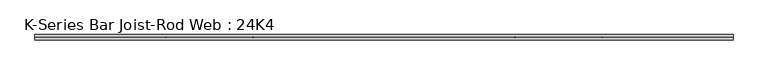
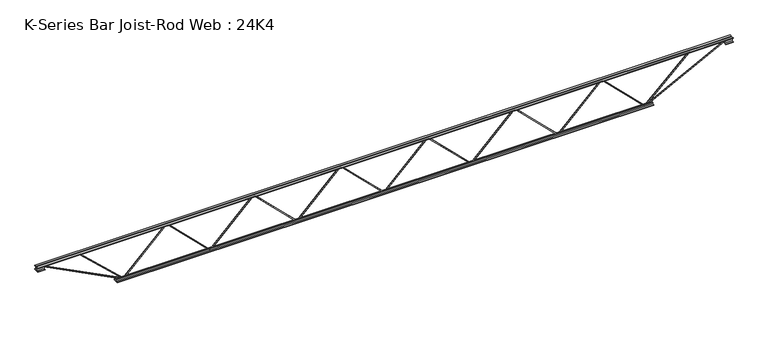
"""IFC4 building model written with IfcOpenShell, lengths in millimetres: beam geometry, K-Series Bar Joist-Rod Web : 24K4."""

from ifc_helpers import new_model, si_unit, frame, origin, place, context, project, spatial, polyline, outline, extrude, source, transform, mapped, element, save


def k_series_bar_joist_rod_web_24k4_b54f82ce(model_context):
    return source(origin(), model_context, "Body", "SweptSolid", [
        extrude(outline(polyline([(-293.6875, 1223.645), (-303.2125, 1223.645), (-303.2125, 1228.7733784), (293.6875, 1834.0077534), (293.6875, 1836.4509966), (-303.2125, 2441.6853716), (-303.2125, 2446.81375), (-293.6875, 2446.81375), (-293.6875, 2445.5921284), (303.2125, 1840.3577534), (303.2125, 1830.1009966), (-293.6875, 1224.8666216), (-293.6875, 1223.645)])), frame((0.0, -4.7625, 0.0), z_axis=(0.0, 1.0, 0.0), x_axis=(0.0, 0.0, 1.0)), (0.0, 0.0, 1.0), 9.525),
        extrude(outline(polyline([(-293.6875, 0.15875), (-303.2125, 0.15875), (-303.2125, 5.2871284), (293.6875, 610.5215034), (293.6875, 612.9647466), (-303.2125, 1218.1991216), (-303.2125, 1223.3275), (-293.6875, 1223.3275), (-293.6875, 1222.1058784), (303.2125, 616.8715034), (303.2125, 606.6147466), (-293.6875, 1.3803716), (-293.6875, 0.15875)])), frame((0.0, -4.7625, 0.0), z_axis=(0.0, 1.0, 0.0), x_axis=(0.0, 0.0, 1.0)), (0.0, 0.0, 1.0), 9.525),
        extrude(outline(polyline([(-293.6875, -1223.3275), (-303.2125, -1223.3275), (-303.2125, -1218.1991216), (293.6875, -612.9647466), (293.6875, -610.5215034), (-303.2125, -5.2871284), (-303.2125, -0.15875), (-293.6875, -0.15875), (-293.6875, -1.3803716), (303.2125, -606.6147466), (303.2125, -616.8715034), (-293.6875, -1222.1058784), (-293.6875, -1223.3275)])), frame((0.0, -4.7625, 0.0), z_axis=(0.0, 1.0, 0.0), x_axis=(0.0, 0.0, 1.0)), (0.0, 0.0, 1.0), 9.525),
        extrude(outline(polyline([(-293.6875, -2446.81375), (-303.2125, -2446.81375), (-303.2125, -2441.6853716), (293.6875, -1836.4509966), (293.6875, -1834.0077534), (-303.2125, -1228.7733784), (-303.2125, -1223.645), (-293.6875, -1223.645), (-293.6875, -1224.8666216), (303.2125, -1830.1009966), (303.2125, -1840.3577534), (-293.6875, -2445.5921284), (-293.6875, -2446.81375)])), frame((0.0, -4.7625, 0.0), z_axis=(0.0, 1.0, 0.0), x_axis=(0.0, 0.0, 1.0)), (0.0, 0.0, 1.0), 9.525),
        extrude(outline(polyline([(-293.6875, 2447.13125), (-303.2125, 2447.13125), (-303.2125, 2452.2596284), (293.6875, 3057.4940034), (293.6875, 3059.9372466), (-303.2125, 3665.1716216), (-303.2125, 3670.3), (-293.6875, 3670.3), (-293.6875, 3669.0783784), (303.2125, 3063.8440034), (303.2125, 3053.5872466), (-293.6875, 2448.3528716), (-293.6875, 2447.13125)])), frame((0.0, -4.7625, 0.0), z_axis=(0.0, 1.0, 0.0), x_axis=(0.0, 0.0, 1.0)), (0.0, 0.0, 1.0), 9.525),
        extrude(outline(polyline([(-293.6875, -3670.3), (-303.2125, -3670.3), (-303.2125, -3665.1716216), (293.6875, -3059.9372466), (293.6875, -3057.4940034), (-303.2125, -2452.2596284), (-303.2125, -2447.13125), (-293.6875, -2447.13125), (-293.6875, -2448.3528716), (303.2125, -3053.5872466), (303.2125, -3063.8440034), (-293.6875, -3669.0783784), (-293.6875, -3670.3)])), frame((0.0, -4.7625, 0.0), z_axis=(0.0, 1.0, 0.0), x_axis=(0.0, 0.0, 1.0)), (0.0, 0.0, 1.0), 9.525),
        extrude(outline(polyline([(4.7625, 304.8), (36.5125, 304.8), (36.5125, 298.45), (11.1125, 298.45), (11.1125, 273.05), (4.7625, 273.05), (4.7625, 304.8)])), frame((-4889.5, 0.0, 0.0), z_axis=(1.0, 0.0, 0.0), x_axis=(0.0, 1.0, 0.0)), (0.0, 0.0, 1.0), 9779.0),
        extrude(outline(polyline([(-4.7625, 304.8), (-4.7625, 273.05), (-11.1125, 273.05), (-11.1125, 298.45), (-36.5125, 298.45), (-36.5125, 304.8), (-4.7625, 304.8)])), frame((-4889.5, 0.0, 0.0), z_axis=(1.0, 0.0, 0.0), x_axis=(0.0, 1.0, 0.0)), (0.0, 0.0, 1.0), 9779.0),
        extrude(outline(polyline([(-4.7625, 241.3), (-36.5125, 241.3), (-36.5125, 247.65), (-11.1125, 247.65), (-11.1125, 273.05), (-4.7625, 273.05), (-4.7625, 241.3)])), frame((-4889.5, 0.0, 0.0), z_axis=(1.0, 0.0, 0.0), x_axis=(0.0, 1.0, 0.0)), (0.0, 0.0, 1.0), 101.6),
        extrude(outline(polyline([(36.5125, 241.3), (4.7625, 241.3), (4.7625, 273.05), (11.1125, 273.05), (11.1125, 247.65), (36.5125, 247.65), (36.5125, 241.3)])), frame((-4889.5, 0.0, 0.0), z_axis=(1.0, 0.0, 0.0), x_axis=(0.0, 1.0, 0.0)), (0.0, 0.0, 1.0), 101.6),
        extrude(outline(polyline([(4.7625, 241.3), (4.7625, 273.05), (11.1125, 273.05), (11.1125, 247.65), (36.5125, 247.65), (36.5125, 241.3), (4.7625, 241.3)])), frame((4787.9, 0.0, 0.0), z_axis=(1.0, 0.0, 0.0), x_axis=(0.0, 1.0, 0.0)), (0.0, 0.0, 1.0), 101.6),
        extrude(outline(polyline([(-4.7625, 241.3), (-36.5125, 241.3), (-36.5125, 247.65), (-11.1125, 247.65), (-11.1125, 273.05), (-4.7625, 273.05), (-4.7625, 241.3)])), frame((4787.9, 0.0, 0.0), z_axis=(1.0, 0.0, 0.0), x_axis=(0.0, 1.0, 0.0)), (0.0, 0.0, 1.0), 101.6),
        extrude(outline(polyline([(4.7625, -304.8), (4.7625, -273.05), (11.1125, -273.05), (11.1125, -298.45), (36.5125, -298.45), (36.5125, -304.8), (4.7625, -304.8)])), frame((-3771.9, 0.0, 0.0), z_axis=(1.0, 0.0, 0.0), x_axis=(0.0, 1.0, 0.0)), (0.0, 0.0, 1.0), 7543.8),
        extrude(outline(polyline([(-4.7625, -304.8), (-36.5125, -304.8), (-36.5125, -298.45), (-11.1125, -298.45), (-11.1125, -273.05), (-4.7625, -273.05), (-4.7625, -304.8)])), frame((-3771.9, 0.0, 0.0), z_axis=(1.0, 0.0, 0.0), x_axis=(0.0, 1.0, 0.0)), (0.0, 0.0, 1.0), 7543.8),
        extrude(outline(polyline([(0.0, -9.525), (0.0, 0.0), (1255.2457966, 0.0), (1255.2457966, -9.525), (0.0, -9.525)])), frame((-4790.0683154, 4.7625, 268.8097388), z_axis=(0.4552893158665215, 0.0, 0.8903435510283628), x_axis=(0.8903435510283628, 0.0, -0.4552893158665215)), (0.0, 0.0, 1.0), 9.525),
        extrude(outline(polyline([(0.0, -9.525), (0.0, 0.0), (837.0470105, 0.0), (837.0470105, -9.525), (0.0, -9.525)])), frame((-4285.1360069, 4.7625, 269.5703023), z_axis=(0.6827573515565594, 0.0, 0.7306451935758373), x_axis=(0.7306451935758373, 0.0, -0.6827573515565594)), (0.0, 0.0, 1.0), 9.525),
        extrude(outline(polyline([(0.0, -9.525), (0.0, 0.0), (1255.2457966, 0.0), (1255.2457966, -9.525), (0.0, -9.525)])), frame((4790.0683154, -4.7625, 268.8097388), z_axis=(-0.455289315866513, 0.0, 0.8903435510283672), x_axis=(-0.8903435510283672, 0.0, -0.455289315866513)), (0.0, 0.0, 1.0), 9.525),
        extrude(outline(polyline([(0.0, -9.525), (0.0, 0.0), (837.0470105, 0.0), (837.0470105, -9.525), (0.0, -9.525)])), frame((4285.1360069, -4.7625, 269.5703023), z_axis=(-0.6827573515565561, 0.0, 0.7306451935758403), x_axis=(-0.7306451935758403, 0.0, -0.6827573515565561)), (0.0, 0.0, 1.0), 9.525),
    ])


if __name__ == "__main__":
    model = new_model("IFC4")
    model_context = context("Model", 3, world=origin())
    ifc_project = project(units=[si_unit("LENGTHUNIT", "METRE", prefix="MILLI")], contexts=[model_context])
    site = spatial("IfcSite", under=ifc_project)
    building = spatial("IfcBuilding", under=site)
    placement = place(None, origin())
    k_series_bar_joist_rod_web_24k4_shape = k_series_bar_joist_rod_web_24k4_b54f82ce(model_context)
    element("IfcBeam", 1, ObjectType="K-Series Bar Joist-Rod Web : 24K4", at=placement, inside=building, context=model_context, shape_type="MappedRepresentation", body=[
        mapped(k_series_bar_joist_rod_web_24k4_shape, transform((0.0, 0.0, 0.0), x_axis=(1.0, 0.0, 0.0), y_axis=(0.0, 1.0, 0.0), z_axis=(0.0, 0.0, 1.0))),
    ])
    save(model, "model.ifc")

# Revit data of these elements
# Type "K-Series Bar Joist-Rod Web : 24K4"
#   Assembly Code = "B1010350"
#   Wt = 8.4
#   Web Thickness = 9.525 mm
#   Start Offset [instance default] = 0 mm
#   Start Extension [instance default] = 0 mm
#   Seat Length = 101.6 mm
#   Seat Depth = 63.5 mm
#   PanelArrayLength [instance default] = 4876.8 mm
#   Panel [instance default] = 1219.2 mm
#   End Offset [instance default] = 0 mm
#   End Extension [instance default] = 0 mm
#   End Panel = 1219.2 mm
#   Cord Leg = 31.75 mm
#   Chord Thickness = 6.35 mm
#   Length [instance default] = 7315.2 mm
#   Depth = 609.6 mm
#   PanelArrayNum [instance default] = 4
#   Structural Material = Steel ASTM A500, Grade C, Round
# Element 1 (IfcBeam, "K-Series Bar Joist-Rod Web : 24K4")
#   PanelArrayLength = 7339.013 mm
#   Panel = 1223.169 mm
#   PanelArrayNum = 6
#   Materials on its faces: "Steel ASTM A500, Grade C, Round"
# Materials
#   "Steel ASTM A500, Grade C, Round": class "Metal", colour RGB 202 101 0, transparency 0, Description = "Carbon steel", Cost = 0
